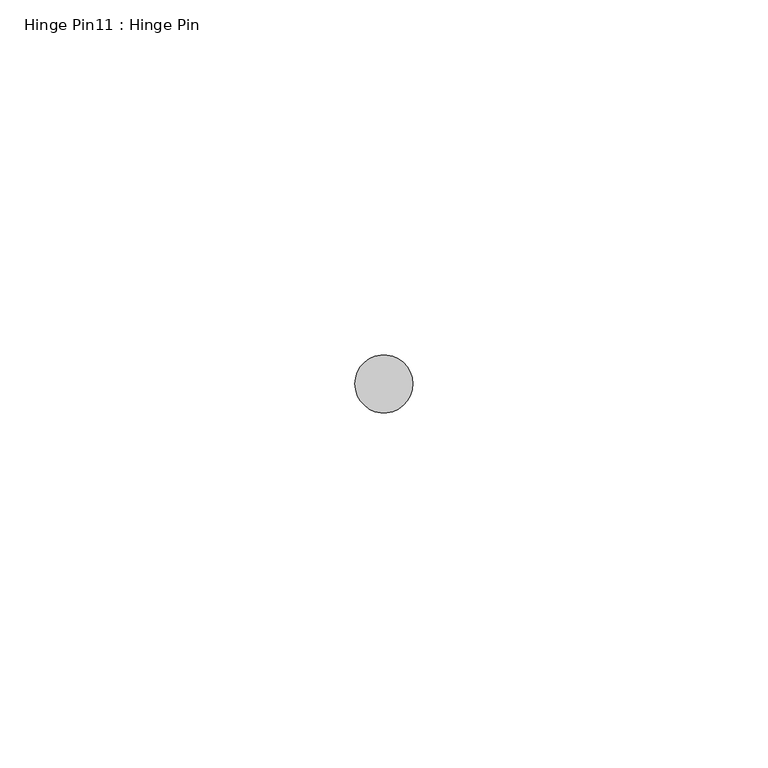
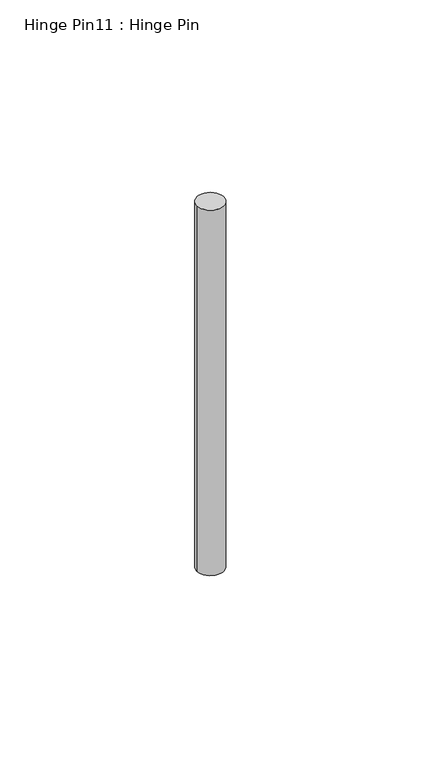
"""IFC4 building model written with IfcOpenShell, lengths in millimetres: proxy geometry, Hinge Pin11 : Hinge Pin."""

from ifc_helpers import new_model, si_unit, point, frame, frame_2d, origin, place, context, project, spatial, circle_curve, trimmed, segment, composite_curve, outline, extrude, source, transform, mapped, element, save


def hinge_pin11_hinge_pin_2f9686dc(model_context):
    return source(origin(), model_context, "Body", "SweptSolid", [
        extrude(outline(composite_curve([segment(trimmed(circle_curve(frame_2d((587319.1320739, -536310.3652841)), 4.0894), [point((587315.0426739, -536310.3652841))], [point((587323.2214739, -536310.3652841))], False, "CARTESIAN"), True, "CONTINUOUS"), segment(trimmed(circle_curve(frame_2d((587319.1320739, -536310.3652841)), 4.0894), [point((587323.2214739, -536310.3652841))], [point((587315.0426739, -536310.3652841))], False, "CARTESIAN"), True, "CONTINUOUS")], self_intersect=False)), frame((0.0, 0.0, 1128.5140625), z_axis=(0.0, 0.0, 1.0), x_axis=(1.0, 0.0, 0.0)), (0.0, 0.0, 1.0), 117.871875),
    ])


if __name__ == "__main__":
    model = new_model("IFC4")
    model_context = context("Model", 3, world=origin())
    ifc_project = project(units=[si_unit("LENGTHUNIT", "METRE", prefix="MILLI")], contexts=[model_context])
    site = spatial("IfcSite", under=ifc_project)
    building = spatial("IfcBuilding", under=site)
    placement = place(None, origin())
    hinge_pin11_hinge_pin_shape = hinge_pin11_hinge_pin_2f9686dc(model_context)
    element("IfcBuildingElementProxy", 1, Name="Hinge Pin11 : Hinge Pin", ObjectType="Hinge Pin11 : Hinge Pin", at=placement, inside=building, context=model_context, shape_type="MappedRepresentation", body=[
        mapped(hinge_pin11_hinge_pin_shape, transform((0.0, 0.0, 0.0), x_axis=(1.0, 0.0, 0.0), y_axis=(0.0, 1.0, 0.0), z_axis=(0.0, 0.0, 1.0))),
    ])
    save(model, "model.ifc")

# Revit data of these elements
# Element 1 (IfcBuildingElementProxy, "Hinge Pin11 : Hinge Pin")
#   Materials on its faces: "6\"X6\" WELD-ON STL BUTT HINGE"
# Materials
#   "6\"X6\" WELD-ON STL BUTT HINGE": class "Metal", colour RGB 189 187 185, transparency 0, Description = "Carbon steel", Cost = 0
